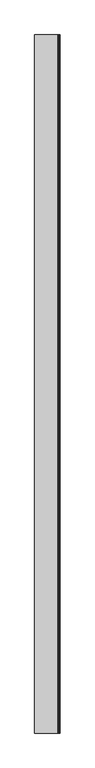
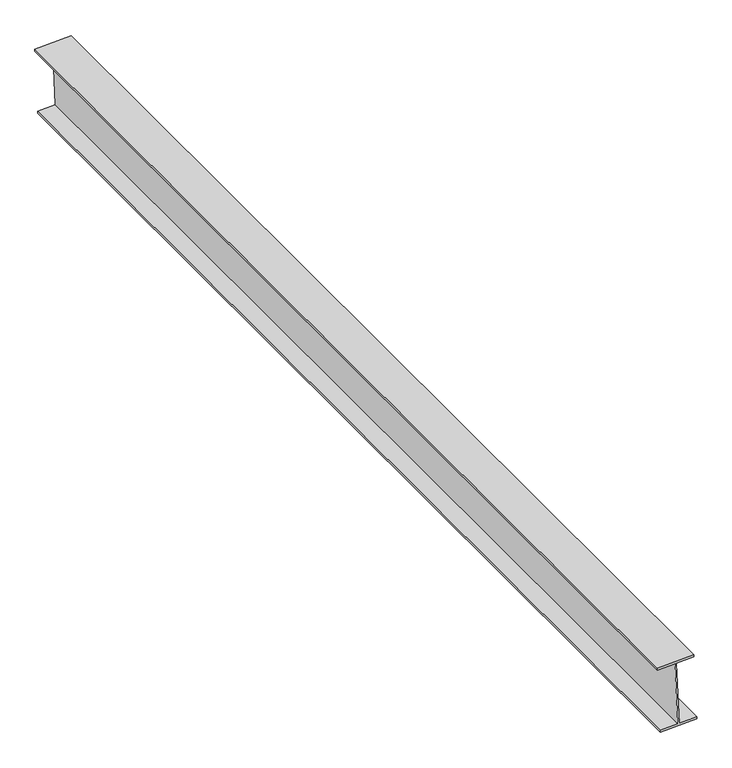
"""IFC4 building model written with IfcOpenShell, lengths in millimetres: proxy geometry, Generic Models 7:Generic Models 1:8:Generic Models 1:8 : Generic Models 7:Generic Models 1:337419:45 : Generic Models 7:Generic Models 1:8:Generic Models 1:8 : Generic Models 7:Generic Models 1:337419:315935."""

from ifc_helpers import new_model, si_unit, frame, origin, place, context, project, spatial, polyline, outline, extrude, source, transform, mapped, element, save


def generic_models_e99133b0(model_context):
    return source(origin(), model_context, "Body", "SweptSolid", [
        extrude(outline(polyline([(3670.9066459, 560594.8242278), (3674.218924, 560674.3189025), (3382.3721534, 560686.4791847), (3379.0598752, 560606.9845098), (3370.1775822, 560607.3546053), (3377.0400533, 560772.0539102), (3385.9223463, 560771.6838146), (3382.6206461, 560692.44301), (3674.4674167, 560680.2827278), (3677.7691169, 560759.5235327), (3686.65141, 560759.1534371), (3679.7889389, 560594.4541323), (3670.9066459, 560594.8242278)])), frame((0.0, -548060.3163841, 0.0), z_axis=(0.0, 1.0, 0.0), x_axis=(0.0, 0.0, 1.0)), (0.0, 0.0, 1.0), 4876.8),
    ])


if __name__ == "__main__":
    model = new_model("IFC4")
    model_context = context("Model", 3, world=origin())
    ifc_project = project(units=[si_unit("LENGTHUNIT", "METRE", prefix="MILLI")], contexts=[model_context])
    site = spatial("IfcSite", under=ifc_project)
    building = spatial("IfcBuilding", under=site)
    placement = place(None, origin())
    generic_models_shape = generic_models_e99133b0(model_context)
    element("IfcBuildingElementProxy", 1, Name="Generic Models 7:Generic Models 1:8:Generic Models 1:8 : Generic Models 7:Generic Models 1:337419:45 : Generic Models 7:Generic Models 1:8:Generic Models 1:8 : Generic Models 7:Generic Models 1:337419:315935", ObjectType="Generic Models 7:Generic Models 1:8:Generic Models 1:8 : Generic Models 7:Generic Models 1:337419:45 : Generic Models 7:Generic Models 1:8:Generic Models 1:8 : Generic Models 7:Generic Models 1:337419:315935", at=placement, inside=building, context=model_context, shape_type="MappedRepresentation", body=[
        mapped(generic_models_shape, transform((0.0, 0.0, 0.0), x_axis=(1.0, 0.0, 0.0), y_axis=(0.0, 1.0, 0.0), z_axis=(0.0, 0.0, 1.0))),
    ])
    save(model, "model.ifc")

# Revit data of these elements
# Type "Generic Models 7:Generic Models 1:8:Generic Models 1:8 : Generic Models 7:Generic Models 1:337419:45 : Generic Models 7:Generic Models 1:8:Generic Models 1:8 : Generic Models 7:Generic Models 1:337419:315935"
#   NameOverride = "Generic Models 7:Generic Models 1:8:Generic Models 1:8 : Generic Models 7:Generic Models 1:337419:315935"
#   ObjectTypeOverride = "Generic Models 1:8 : Generic Models 7:Generic Models 1:337419"
#   Reference = "Generic Models 1"
#   Tag = "315935"
# Element 1 (IfcBuildingElementProxy, "Generic Models 7:Generic Models 1:8:Generic Models 1:8 : Generic Models 7:Generic Models 1:337419:45 : Generic Models 7:Generic Models 1:8:Generic Models 1:8 : Generic Models 7:Generic Models 1:337419:315935")
#   Materials on its faces: "STRUCTURAL STEEL - SEE STRUCT. DWGS"
# Materials
#   "STRUCTURAL STEEL - SEE STRUCT. DWGS": class "Metal", colour RGB 189 187 185, transparency 0, Description = "Structural steel 50ksi", Cost = 0
